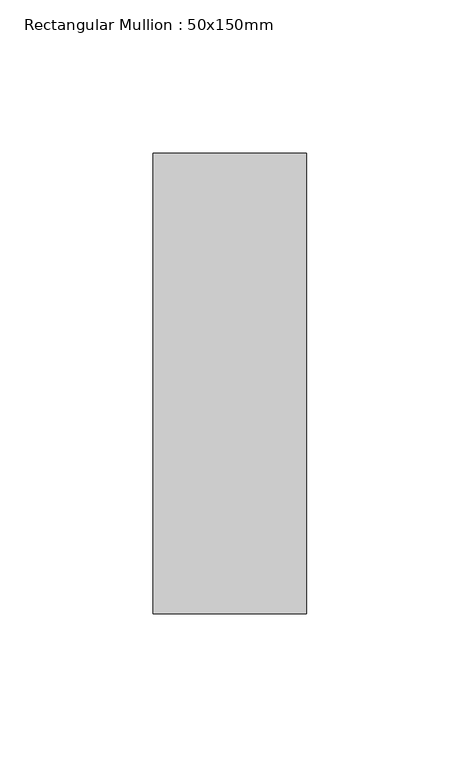
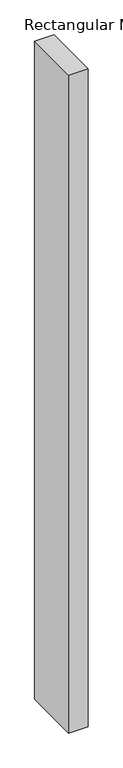
"""IFC4 building model written with IfcOpenShell, lengths in millimetres: member geometry, Rectangular Mullion : 50x150mm."""

from ifc_helpers import new_model, si_unit, frame, origin, place, context, project, spatial, polyline, outline, extrude, source, transform, mapped, element, save


def rectangular_mullion_50x150mm_f5b8645b(model_context):
    return source(origin(), model_context, "Body", "SweptSolid", [
        extrude(outline(polyline([(25.0, 75.0), (25.0, -75.0), (-25.0, -75.0), (-25.0, 75.0), (25.0, 75.0)])), frame((0.0, 0.0, -1780.0), z_axis=(0.0, 0.0, 1.0), x_axis=(1.0, 0.0, 0.0)), (0.0, 0.0, 1.0), 1780.0),
    ])


if __name__ == "__main__":
    model = new_model("IFC4")
    model_context = context("Model", 3, world=origin())
    ifc_project = project(units=[si_unit("LENGTHUNIT", "METRE", prefix="MILLI")], contexts=[model_context])
    site = spatial("IfcSite", under=ifc_project)
    building = spatial("IfcBuilding", under=site)
    placement = place(None, origin())
    rectangular_mullion_50x150mm_shape = rectangular_mullion_50x150mm_f5b8645b(model_context)
    element("IfcMember", 1, ObjectType="Rectangular Mullion : 50x150mm", at=placement, inside=building, context=model_context, shape_type="MappedRepresentation", body=[
        mapped(rectangular_mullion_50x150mm_shape, transform((0.0, 0.0, 0.0), x_axis=(1.0, 0.0, 0.0), y_axis=(0.0, 1.0, 0.0), z_axis=(0.0, 0.0, 1.0))),
    ])
    save(model, "model.ifc")

# Revit data of these elements
# Type "Rectangular Mullion : 50x150mm"
#   Keynote = "H11"
#   built-in parameter 1007304 = 0.492126 (stored number, unit not read)
#   built-in parameter 1007301 = 0.082021 (stored number, unit not read)
#   built-in parameter 1007300 = 0.082021 (stored number, unit not read)
# Element 1 (IfcMember, "Rectangular Mullion : 50x150mm")
#   Materials on its faces: "Aluminium"
# Materials
#   "Aluminium": class "Metal", colour RGB 247 247 247, transparency 0, Description = "Aluminium 6061", Cost = 0
